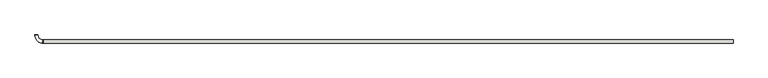
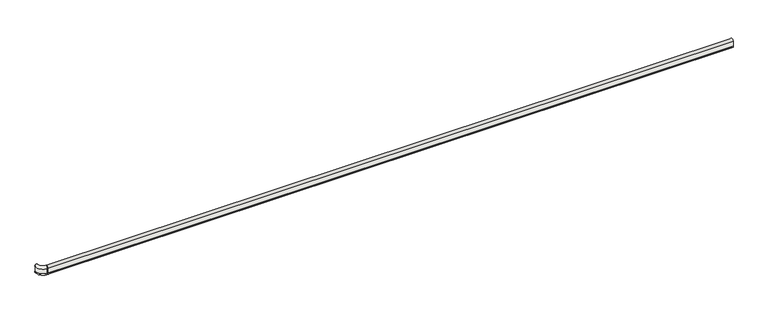
"""IFC4 building model written with IfcOpenShell, lengths in millimetres: covering geometry, Construction_Railing_SPM_Starline-Anodisee-Decowood : Decowood."""

import ifcopenshell
import ifcopenshell.guid

model = None  # the IFC model being written
_history = None  # IfcOwnerHistory: only IFC2X3 demands one
_inside = {}  # id of a spatial element -> (the spatial element, [elements in it])
_under = {}  # id of a project, library or spatial element -> (it, [spatial elements below it])
_declared = {}  # id of a project -> (the project, [libraries it declares])
_typed = {}  # id of a type object -> (the type object, [elements of that type])
_made_of = {}  # id of a material, layer set ... -> (it, [elements and type objects made of it])


def new_model(schema):
    """Start an empty IFC model of exactly this schema.

    Asked for "IFC4X3", IfcOpenShell would pick the latest addendum, in which some entities
    have other attributes; the version numbers below select the first issue.
    IFC2X3 requires an IfcOwnerHistory on every rooted entity: one is made here for all.
    """
    global model, _history
    if schema == "IFC4X3":
        model = ifcopenshell.file(schema_version=(4, 3, 0, 0))
    else:
        model = ifcopenshell.file(schema=schema)
    _inside.clear()
    _under.clear()
    _declared.clear()
    _typed.clear()
    _made_of.clear()
    _history = None
    if model.schema == "IFC2X3":
        org = make("IfcOrganization", Name="unknown")
        user = make(
            "IfcPersonAndOrganization",
            ThePerson=make("IfcPerson", FamilyName="unknown"),
            TheOrganization=org,
        )
        app = make(
            "IfcApplication",
            ApplicationDeveloper=org,
            Version="unknown",
            ApplicationFullName="unknown",
            ApplicationIdentifier="unknown",
        )
        _history = make(
            "IfcOwnerHistory",
            OwningUser=user,
            OwningApplication=app,
            ChangeAction="ADDED",
            CreationDate=0,
        )
    return model


def make(cls, **values):
    """One entity of the class cls with the attributes given. An attribute that is None is left unset."""
    return model.create_entity(
        cls, **{name: value for name, value in values.items() if value is not None}
    )


def rooted(cls, **values):
    """An entity with a GlobalId (a new one), such as an element, a storey or a relation."""
    return make(cls, GlobalId=ifcopenshell.guid.new(), OwnerHistory=_history, **values)


def si_unit(unit_type, name, prefix=None):
    """IfcSIUnit, for example si_unit("LENGTHUNIT", "METRE", prefix="MILLI")."""
    return make("IfcSIUnit", UnitType=unit_type, Prefix=prefix, Name=name)


def assignment(units):
    """IfcUnitAssignment: the units of a project."""
    return None if units is None else make("IfcUnitAssignment", Units=units)


def point(xyz):
    """IfcCartesianPoint."""
    return None if xyz is None else make("IfcCartesianPoint", Coordinates=xyz)


def direction(xyz):
    """IfcDirection."""
    return None if xyz is None else make("IfcDirection", DirectionRatios=xyz)


def frame(location, z_axis=None, x_axis=None):
    """IfcAxis2Placement3D, a coordinate frame: its origin and axes. An axis left out is left unset."""
    return make(
        "IfcAxis2Placement3D",
        Location=point(location),
        Axis=direction(z_axis),
        RefDirection=direction(x_axis),
    )


def frame_2d(location, x_axis=None):
    """IfcAxis2Placement2D, a coordinate frame in the plane: its origin and x axis."""
    return make(
        "IfcAxis2Placement2D", Location=point(location), RefDirection=direction(x_axis)
    )


def origin():
    """The frame at (0, 0, 0) with its axes left unset."""
    return frame((0.0, 0.0, 0.0))


def place(relative_to, where):
    """IfcLocalPlacement: puts the frame where relative to a parent placement (None: the world)."""
    return make(
        "IfcLocalPlacement", PlacementRelTo=relative_to, RelativePlacement=where
    )


def context(
    kind, dimensions, precision=None, world=None, true_north=None, identifier=None
):
    """IfcGeometricRepresentationContext, for example the 3D "Model" context."""
    return make(
        "IfcGeometricRepresentationContext",
        ContextIdentifier=identifier,
        ContextType=kind,
        CoordinateSpaceDimension=dimensions,
        Precision=precision,
        WorldCoordinateSystem=world,
        TrueNorth=true_north,
    )


def project(units=None, contexts=None):
    """IfcProject with its units and contexts."""
    return rooted(
        "IfcProject",
        Name="project",
        RepresentationContexts=contexts,
        UnitsInContext=assignment(units),
    )


def spatial(cls, under=None, at=None, **own):
    """A site, building, storey or space (cls), placed at a placement, below another one or the project."""
    s = rooted(cls, ObjectPlacement=at, **own)
    if under is not None:
        _under.setdefault(under.id(), (under, []))[1].append(s)
    return s


def polyline(points):
    """IfcPolyline through the points."""
    return make("IfcPolyline", Points=[point(p) for p in points])


def circle_curve(where, radius):
    """IfcCircle in the frame where."""
    return make("IfcCircle", Position=where, Radius=radius)


def ellipse_curve(where, semi_axis1, semi_axis2):
    """IfcEllipse in the frame where."""
    return make(
        "IfcEllipse", Position=where, SemiAxis1=semi_axis1, SemiAxis2=semi_axis2
    )


def trimmed(basis, trim1, trim2, sense, master):
    """IfcTrimmedCurve: the piece of a basis curve between two trims."""
    return make(
        "IfcTrimmedCurve",
        BasisCurve=basis,
        Trim1=trim1,
        Trim2=trim2,
        SenseAgreement=sense,
        MasterRepresentation=master,
    )


def segment(curve, same_sense, transition):
    """IfcCompositeCurveSegment."""
    return make(
        "IfcCompositeCurveSegment",
        Transition=transition,
        SameSense=same_sense,
        ParentCurve=curve,
    )


def composite_curve(segments, self_intersect=None):
    """IfcCompositeCurve: segments joined end to end."""
    return make("IfcCompositeCurve", Segments=segments, SelfIntersect=self_intersect)


def outline(outer, holes=None, kind="AREA"):
    """IfcArbitraryClosedProfileDef: a profile drawn as a closed curve; with holes, ...WithVoids."""
    if holes is None:
        return make("IfcArbitraryClosedProfileDef", ProfileType=kind, OuterCurve=outer)
    return make(
        "IfcArbitraryProfileDefWithVoids",
        ProfileType=kind,
        OuterCurve=outer,
        InnerCurves=holes,
    )


def extrude(swept, where, along, depth):
    """IfcExtrudedAreaSolid: the profile swept, set in the frame where, extruded along a direction by depth."""
    return make(
        "IfcExtrudedAreaSolid",
        SweptArea=swept,
        Position=where,
        ExtrudedDirection=direction(along),
        Depth=depth,
    )


def shape(context_of_items, identifier, shape_type, items):
    """IfcShapeRepresentation: the items that make up one representation, for example the "Body"."""
    return make(
        "IfcShapeRepresentation",
        ContextOfItems=context_of_items,
        RepresentationIdentifier=identifier,
        RepresentationType=shape_type,
        Items=items,
    )


def source(mapping_origin, context_of_items, identifier, shape_type, items):
    """IfcRepresentationMap: a shape defined once, which mapped items show again and again."""
    return make(
        "IfcRepresentationMap",
        MappingOrigin=mapping_origin,
        MappedRepresentation=shape(context_of_items, identifier, shape_type, items),
    )


def transform(
    local_origin,
    x_axis=None,
    y_axis=None,
    z_axis=None,
    scale=None,
    scale2=None,
    scale3=None,
    uniform=True,
):
    """IfcCartesianTransformationOperator3D, or its non-uniform kind. x_axis, y_axis, z_axis: its Axis1, 2, 3."""
    if uniform:
        return make(
            "IfcCartesianTransformationOperator3D",
            Axis1=direction(x_axis),
            Axis2=direction(y_axis),
            LocalOrigin=point(local_origin),
            Scale=scale,
            Axis3=direction(z_axis),
        )
    return make(
        "IfcCartesianTransformationOperator3DnonUniform",
        Axis1=direction(x_axis),
        Axis2=direction(y_axis),
        LocalOrigin=point(local_origin),
        Scale=scale,
        Axis3=direction(z_axis),
        Scale2=scale2,
        Scale3=scale3,
    )


def mapped(mapping_source, mapping_target):
    """IfcMappedItem: shows the shape of a source again, moved by a transform."""
    return make(
        "IfcMappedItem", MappingSource=mapping_source, MappingTarget=mapping_target
    )


def made_of(thing, what):
    """Note that an element or type object is made of a material, layer set ...; save() writes the relation."""
    if what is not None:
        _made_of.setdefault(what.id(), (what, []))[1].append(thing)
    return thing


def element(
    cls,
    number,
    at=None,
    inside=None,
    cuts=None,
    type_object=None,
    material=None,
    context=None,
    identifier="Body",
    shape_type=None,
    held_by="IfcProductDefinitionShape",
    body=None,
    shapes=None,
    **own,
):
    """One element of the class cls, such as IfcWall. Its Tag is "e" and its number.

    at: its placement. inside: the storey or other place that contains it. cuts: it is an
    opening in that element (IfcRelVoidsElement). A single representation is given by context,
    identifier, shape_type and body (its items); several are given by shapes. held_by: the class
    of the entity that holds the representations. save() writes the other relations.
    """
    e = rooted(cls, Tag="e%d" % number, ObjectPlacement=at, **own)
    if body is not None:
        shapes = [shape(context, identifier, shape_type, body)]
    if shapes is not None:
        e.Representation = make(held_by, Representations=shapes)
    if inside is not None:
        _inside.setdefault(inside.id(), (inside, []))[1].append(e)
    if cuts is not None:
        rooted(
            "IfcRelVoidsElement", RelatingBuildingElement=cuts, RelatedOpeningElement=e
        )
    if type_object is not None:
        _typed.setdefault(type_object.id(), (type_object, []))[1].append(e)
    return made_of(e, material)


def aggregate(whole, parts):
    """IfcRelAggregates: a whole, such as a stair, and the parts it consists of."""
    return rooted("IfcRelAggregates", RelatingObject=whole, RelatedObjects=parts)


def save(model, path):
    """Write the relations noted so far, then the file.

    IfcRelAggregates (storeys below a building ...), IfcRelContainedInSpatialStructure (elements
    in a storey), IfcRelDefinesByType, IfcRelAssociatesMaterial and IfcRelDeclares: one each for
    every whole, place, type object, material and project.
    """
    for whole, parts in _under.values():
        aggregate(whole, parts)
    for where, things in _inside.values():
        rooted(
            "IfcRelContainedInSpatialStructure",
            RelatedElements=things,
            RelatingStructure=where,
        )
    for kind, things in _typed.values():
        rooted("IfcRelDefinesByType", RelatedObjects=things, RelatingType=kind)
    for what, things in _made_of.values():
        rooted("IfcRelAssociatesMaterial", RelatedObjects=things, RelatingMaterial=what)
    for by, libraries in _declared.values():
        rooted("IfcRelDeclares", RelatingContext=by, RelatedDefinitions=libraries)
    model.write(path)


def plane_surface(at):
    """IfcPlane: the flat surface through the origin of the frame at, square to its z axis."""
    return make("IfcPlane", Position=at)


def cylinder_surface(at, radius):
    """IfcCylindricalSurface: all points at the distance radius from the z axis of the frame at."""
    return make("IfcCylindricalSurface", Position=at, Radius=radius)


def revolved_surface(curve, axis_point, axis_direction):
    """IfcSurfaceOfRevolution: the curve turned about the line through axis_point along axis_direction."""
    return make(
        "IfcSurfaceOfRevolution",
        SweptCurve=make("IfcArbitraryOpenProfileDef", ProfileType="CURVE", Curve=curve),
        AxisPosition=make("IfcAxis1Placement", Location=point(axis_point), Axis=direction(axis_direction)),
    )


def advanced_brep(points, edges, surfaces, faces):
    """IfcAdvancedBrep: a solid bounded by faces that lie on surfaces and meet in shared edges.

    An edge is (start, end): straight between two places in points (the first is 0);
    or (start, end, curve); or (start, end, curve, False) where it runs against its curve.
    A face is (place in surfaces, loops), or (place, loops, False) where it looks against
    its surface's normal. A loop lists edges by number (the first is 1), with a minus sign
    where the edge is run from its end to its start. The first loop is the outer one.
    """
    corners = [point(p) for p in points]
    vertices = [make("IfcVertexPoint", VertexGeometry=c) for c in corners]
    made = []
    for start, end, *more in edges:
        made.append(
            make(
                "IfcEdgeCurve",
                EdgeStart=vertices[start],
                EdgeEnd=vertices[end],
                EdgeGeometry=more[0] if more else make("IfcPolyline", Points=[corners[start], corners[end]]),
                SameSense=more[1] if len(more) > 1 else True,
            )
        )
    hull = []
    for where, loops, *sense in faces:
        bounds = []
        for j, loop in enumerate(loops):
            ring = [make("IfcOrientedEdge", EdgeElement=made[abs(k) - 1], Orientation=k > 0) for k in loop]
            bounds.append(
                make(
                    "IfcFaceOuterBound" if j == 0 else "IfcFaceBound",
                    Bound=make("IfcEdgeLoop", EdgeList=ring),
                    Orientation=True,
                )
            )
        hull.append(make("IfcAdvancedFace", Bounds=bounds, FaceSurface=surfaces[where], SameSense=sense[0] if sense else True))
    return make("IfcAdvancedBrep", Outer=make("IfcClosedShell", CfsFaces=hull))


def covering_4a841b85(model_context):
    return source(origin(), model_context, "Body", "SolidModel", [
        advanced_brep(
        [(0.0, -52.1949146, 777.1298269), (0.0, -78.97282, 779.8387167), (0.0, -77.7797808, 779.8387167), (0.0, -77.7797808, 730.187687), (0.0, -79.0444967, 730.187687), (0.0, -52.1949146, 732.7970729), (-1.0, -52.1949146, 777.1298269), (-1.0, -78.97282, 779.8387167), (-78.97282, -1.0, 779.8387167), (-78.97282, 0.0, 779.8387167), (-77.7797808, 0.0, 779.8387167), (-77.7797808, -1.0, 779.8387167), (-1.0, -77.7797808, 779.8387167), (-1.0, -77.7797808, 730.187687), (-77.7797808, -1.0, 730.187687), (-77.7797808, 0.0, 730.187687), (-79.0444967, 0.0, 730.187687), (-79.0444967, -1.0, 730.187687), (-1.0, -79.0444967, 730.187687), (-1.0, -52.1949146, 732.7970729), (-52.1949146, -1.0, 777.1298269), (-52.1949146, -1.0, 732.7970729), (-52.1949146, 0.0, 777.1298269), (-52.1949146, 0.0, 732.7970729)],
        [
            (0, 1, circle_curve(frame((0.0, -64.921376, 785.0331273), z_axis=(1.0, 0.0, 0.0), x_axis=(0.0, -1.0, 0.0)), 14.9808204)),
            (1, 2),
            (2, 3),
            (3, 4),
            (4, 5, circle_curve(frame((0.0, -64.9833199, 724.9442146), z_axis=(1.0, 0.0, 0.0), x_axis=(0.0, -1.0, 0.0)), 15.0070215)),
            (5, 0),
            (0, 6),
            (6, 7, circle_curve(frame((-1.0, -64.921376, 785.0331273), z_axis=(1.0, 0.0, 0.0), x_axis=(0.0, -1.0, 0.0)), 14.9808204)),
            (7, 1),
            (7, 8, circle_curve(frame((-1.0, -1.0, 779.8387167), z_axis=(0.0, 0.0, -1.0), x_axis=(0.0, -1.0, 0.0)), 77.97282)),
            (8, 9),
            (9, 10),
            (10, 11),
            (11, 12, circle_curve(frame((-1.0, -1.0, 779.8387167), z_axis=(0.0, 0.0, 1.0), x_axis=(0.0, -1.0, 0.0)), 76.7797808)),
            (12, 2),
            (12, 13),
            (13, 3),
            (13, 14, circle_curve(frame((-1.0, -1.0, 730.187687), z_axis=(0.0, 0.0, -1.0), x_axis=(0.0, -1.0, 0.0)), 76.7797808)),
            (14, 15),
            (15, 16),
            (16, 17),
            (17, 18, circle_curve(frame((-1.0, -1.0, 730.187687), z_axis=(0.0, 0.0, 1.0), x_axis=(0.0, -1.0, 0.0)), 78.0444967)),
            (18, 4),
            (18, 19, circle_curve(frame((-1.0, -64.9833199, 724.9442146), z_axis=(1.0, 0.0, 0.0), x_axis=(0.0, -1.0, 0.0)), 15.0070215)),
            (19, 5),
            (19, 6),
            (6, 20, circle_curve(frame((-1.0, -1.0, 777.1298269), z_axis=(0.0, 0.0, -1.0), x_axis=(0.0, -1.0, 0.0)), 51.1949146)),
            (20, 8, circle_curve(frame((-64.921376, -1.0, 785.0331273), z_axis=(0.0, -1.0, 0.0), x_axis=(-1.0, 0.0, 0.0)), 14.9808204)),
            (11, 14),
            (21, 19, circle_curve(frame((-1.0, -1.0, 732.7970729), z_axis=(0.0, 0.0, 1.0), x_axis=(0.0, -1.0, 0.0)), 51.1949146)),
            (17, 21, circle_curve(frame((-64.9833199, -1.0, 724.9442146), z_axis=(0.0, -1.0, 0.0), x_axis=(-1.0, 0.0, 0.0)), 15.0070215)),
            (21, 20),
            (22, 23),
            (23, 16, circle_curve(frame((-64.9833199, 0.0, 724.9442146), z_axis=(0.0, 1.0, 0.0), x_axis=(-1.0, 0.0, 0.0)), 15.0070215)),
            (15, 10),
            (9, 22, circle_curve(frame((-64.921376, 0.0, 785.0331273), z_axis=(0.0, 1.0, 0.0), x_axis=(-1.0, 0.0, 0.0)), 14.9808204)),
            (20, 22),
            (23, 21),
        ],
        [
            plane_surface(frame((0.0, -50.0, 710.0), z_axis=(1.0, 0.0, 0.0), x_axis=(0.0, 0.0, 1.0))),
            cylinder_surface(frame((0.0, -64.921376, 785.0331273), z_axis=(1.0, 0.0, 0.0), x_axis=(0.0, -1.0, 0.0)), 14.9808204),
            plane_surface(frame((0.0, -78.97282, 779.8387167), z_axis=(0.0, 0.0, -1.0), x_axis=(-1.0, 0.0, 0.0))),
            plane_surface(frame((0.0, -77.7797808, 779.8387167), z_axis=(0.0, -1.0, 0.0), x_axis=(-1.0, 0.0, 0.0))),
            plane_surface(frame((0.0, -77.7797808, 730.187687), z_axis=(0.0, 0.0, 1.0), x_axis=(-1.0, 0.0, 0.0))),
            cylinder_surface(frame((0.0, -64.9833199, 724.9442146), z_axis=(1.0, 0.0, 0.0), x_axis=(0.0, -1.0, 0.0)), 15.0070215),
            plane_surface(frame((0.0, -52.1949146, 732.7970729), z_axis=(0.0, 1.0, 0.0), x_axis=(-1.0, 0.0, 0.0))),
            revolved_surface(trimmed(ellipse_curve(frame((-1.0, -64.921376, 785.0331273), z_axis=(1.0, 0.0, 0.0), x_axis=(0.0, -1.0, 0.0)), 14.9808204, 14.9808204), [point((-1.0, -52.1949146, 777.1298269))], [point((-1.0, -78.97282, 779.8387167))], True, "CARTESIAN"), (-1.0, -1.0, 710.0), (0.0, 0.0, -1.0)),
            cylinder_surface(frame((-1.0, -1.0, 710.0), z_axis=(0.0, 0.0, -1.0), x_axis=(0.0, -1.0, 0.0)), 76.7797808),
            revolved_surface(trimmed(ellipse_curve(frame((-1.0, -64.9833199, 724.9442146), z_axis=(1.0, 0.0, 0.0), x_axis=(0.0, -1.0, 0.0)), 15.0070215, 15.0070215), [point((-1.0, -79.0444967, 730.187687))], [point((-1.0, -52.1949146, 732.7970729))], True, "CARTESIAN"), (-1.0, -1.0, 710.0), (0.0, 0.0, -1.0)),
            revolved_surface(polyline([(-1.0, -52.1949146, 732.7970729), (-1.0, -52.1949146, 777.1298269)]), (-1.0, -1.0, 710.0), (0.0, 0.0, -1.0)),
            plane_surface(frame((-50.0, 0.0, 710.0), z_axis=(0.0, 1.0, 0.0), x_axis=(0.0, 0.0, 1.0))),
            cylinder_surface(frame((-64.921376, -1.0, 785.0331273), z_axis=(0.0, -1.0, 0.0), x_axis=(-1.0, 0.0, 0.0)), 14.9808204),
            plane_surface(frame((-77.7797808, -1.0, 779.8387167), z_axis=(-1.0, 0.0, 0.0), x_axis=(0.0, 1.0, 0.0))),
            cylinder_surface(frame((-64.9833199, -1.0, 724.9442146), z_axis=(0.0, -1.0, 0.0), x_axis=(-1.0, 0.0, 0.0)), 15.0070215),
            plane_surface(frame((-52.1949146, -1.0, 732.7970729), z_axis=(1.0, 0.0, 0.0), x_axis=(0.0, 1.0, 0.0))),
        ],
        [
            (0, [[1, 2, 3, 4, 5, 6]]),
            (1, [[-1, 7, 8, 9]]),
            (2, [[-2, -9, 10, 11, 12, 13, 14, 15]]),
            (3, [[-3, -15, 16, 17]]),
            (4, [[-4, -17, 18, 19, 20, 21, 22, 23]]),
            (5, [[-5, -23, 24, 25]]),
            (6, [[-6, -25, 26, -7]]),
            (7, [[-10, -8, 27, 28]]),
            (8, [[-18, -16, -14, 29]]),
            (9, [[30, -24, -22, 31]]),
            (10, [[-27, -26, -30, 32]]),
            (11, [[33, 34, -20, 35, -12, 36]]),
            (12, [[-28, 37, -36, -11]]),
            (13, [[-29, -13, -35, -19]]),
            (14, [[-31, -21, -34, 38]]),
            (15, [[-32, -38, -33, -37]]),
        ],
    ),
        extrude(outline(composite_curve([segment(trimmed(circle_curve(frame_2d((-64.921376, 785.0331273)), 14.9808204), [point((-78.97282, 779.8387167))], [point((-52.1949146, 777.1298269))], False, "CARTESIAN"), True, "CONTINUOUS"), segment(polyline([(-52.1949146, 777.1298269), (-52.1949146, 732.7970729)]), True, "CONTINUOUS"), segment(trimmed(circle_curve(frame_2d((-64.9833199, 724.9442146)), 15.0070215), [point((-52.1949146, 732.7970729))], [point((-79.0444967, 730.187687))], False, "CARTESIAN"), True, "CONTINUOUS"), segment(polyline([(-79.0444967, 730.187687), (-77.7797808, 730.187687), (-77.7797808, 779.8387167), (-78.97282, 779.8387167)]), True, "CONTINUOUS")], self_intersect=False)), frame((0.0, 0.0, 0.0), z_axis=(1.0, 0.0, 0.0), x_axis=(0.0, 1.0, 0.0)), (0.0, 0.0, 1.0), 6800.0),
        extrude(outline(polyline([(0.0, -79.3173438), (0.0, -77.7797808), (6800.0, -77.7797808), (6800.0, -79.3173438), (0.0, -79.3173438)])), frame((0.0, 0.0, 730.187687), z_axis=(0.0, 0.0, 1.0), x_axis=(1.0, 0.0, 0.0)), (0.0, 0.0, 1.0), 49.6510297),
    ])


if __name__ == "__main__":
    model = new_model("IFC4")
    model_context = context("Model", 3, world=origin())
    ifc_project = project(units=[si_unit("LENGTHUNIT", "METRE", prefix="MILLI")], contexts=[model_context])
    site = spatial("IfcSite", under=ifc_project)
    building = spatial("IfcBuilding", under=site)
    placement = place(None, origin())
    covering_shape = covering_4a841b85(model_context)
    element("IfcCovering", 1, ObjectType="Construction_Railing_SPM_Starline-Anodisee-Decowood : Decowood", at=placement, inside=building, context=model_context, shape_type="MappedRepresentation", body=[
        mapped(covering_shape, transform((0.0, 0.0, 0.0), x_axis=(1.0, 0.0, 0.0), y_axis=(0.0, 1.0, 0.0), z_axis=(0.0, 0.0, 1.0))),
    ])
    save(model, "model.ifc")

# Revit data of these elements
# Type "Construction_Railing_SPM_Starline-Anodisee-Decowood : Decowood"
#   WarrantyStartDate [instance default] = "1900-12-31T23:59:59"
#   WarrantyGuarantorParts = "n/a"
#   WarrantyGuarantorLabor = "n/a"
#   WarrantyDurationUnit = "year"
#   WarrantyDurationParts = "n/a"
#   WarrantyDurationLabor = "n/a"
#   WarrantyDescription = "n/a"
#   WallStandoff = "50 mm"
#   URL = "www.spm.fr"
#   UNSPSC Code = ""
#   TagNumber [instance default] = "n/a"
#   SustainabilityPerformance = "n/a"
#   SurfaceSpreadOfFlame = "n/a"
#   Size = "90 x 80 x 4000 mm"
#   Shape = "Elliptical"
#   SerialNumber [instance default] = "n/a"
#   ReplacementCost = "n/a"
#   Reference = "n/a"
#   Projection = "80 mm"
#   Product data url = "http://bimobject.com/spm/product/SPM-STARLINE-DECO"
#   Product Guid = "a7a4224a-4578-432f-a478-06146786615d"
#   OmniClass Description = ""
#   OmniClass Code = ""
#   Name = "WallProtectionPanels_StarlineDecowoodHandrail_GerflorLtd"
#   NBS Reference Description = ""
#   NBS Reference Code = ""
#   ModelReference = "Starline Decowood Handrail"
#   ModelNumber = "n/a"
#   Model = "Starline Decowood Handrail"
#   Material secondary = ""
#   Material main = ""
#   Material = "1.5 mm thick aluminium"
#   Manufacturer = "SPM"
#   Keynote = "09100"
#   InstallationDate [instance default] = "1900-12-31T23:59:59"
#   IfcExportType = "NOTDEFINED"
#   IfcExportAs = "IfcCoveringType"
#   IFC Classification = ""
#   Grade = "n/a"
#   FragilityRating = "n/a"
#   FlammabilityRating = "n/a"
#   Fixing = "2-point self-locking perforated satin silver anodized aluminium brackets"
#   FireRating = "B-s2, d0"
#   Finish = "Aluminium profile: Satin silver anodized; PVC band: Wood effect"
#   Features = "Excellent wrenching resistance, antibacterial"
#   ExpectedLife = "n/a"
#   EnvironmentalProductDeclaration = "n/a"
#   EAN code = ""
#   DurationUnit = "year"
#   Description = "Range only available for the French market"
#   CrossSection = "Elliptical"
#   Constituents = "n/a"
#   ColourOptions = "PVC band: 7 wood effect and 2 trend effect colours available"
#   Color = "n/a"
#   CodePerformance = "n/a"
#   Category = "n/a"
#   COBIe Type Category = ""
#   BarCode [instance default] = "n/a"
#   BIMobject category = ""
#   AssetType = "Fixed"
#   AssetIdentifier [instance default] = "n/a"
#   Assembly Code = "C10"
#   Applications = "Straight and curved corridors in public buildings such as hospitals, clinics, retirement homes, hotels and offices"
#   AcousticRating = "n/a"
#   Accessories = "90° external angle pieces, Variable angles, Wall returns"
#   AccessibilityPerformance = "n/a"
#   Width = 80 mm
#   TotalThickness = 80 mm
#   SpacerOffsetRight [instance default] = 100 mm
#   SpacerOffsetLeft [instance default] = 100 mm
#   OffsetFromWall = 50 mm
#   NominalLength [instance default] = 4000 mm
#   Height = 90 mm
#   HandrailHeight [instance default] = 800 mm
#   SpacerVerticalPlacement [instance default] = 724 mm
#   SpacerCentreToCentreDistance [instance default] = 950 mm
#   SpacerCalc [instance default] = 3800 mm
#   SpacerOffsetRightControl [instance default] = 100 mm
#   SpacerOffsetLeftControl [instance default] = 100 mm
#   MaximumSpacerCentreDistance [instance default] = 1200 mm
#   built-in parameter 1001306 [instance default] = 13.1234 (stored number, unit not read)
#   Diameter = 0 mm
#   Depth = 80 mm
#   NumberOfStandardRailLengths [instance default] = 1
#   NumberOfSpacers [instance default] = 5
#   IsExternal = no
#   HasHeavyTraffic [instance default] = no
#   Edition number = 1
#   CrashRailInternalCornerRight [instance default] = no
#   CrashRailInternalCornerLeft [instance default] = no
#   CrashRailExternalCornerRight [instance default] = yes
#   CrashRailExternalCornerLeft [instance default] = yes
#   CrashRailEndCapRight [instance default] = no
#   CrashRailEndCapLeft [instance default] = no
#   Combustible = no
#   InsertMaterial = PVC - SPM - Erable
#   SpacerMaterial = PVC - SPM - Hêtre
#   RailMaterial = PVC - SPM - Wengé
#   Default Elevation = 0
#   Cost = 0
# Element 1 (IfcCovering, "Construction_Railing_SPM_Starline-Anodisee-Decowood : Decowood")
#   NominalLength = 6800 mm
#   SpacerCentreToCentreDistance = 1100 mm
#   SpacerCalc = 6600 mm
#   built-in parameter 1001306 = 22.3097 (stored number, unit not read)
#   NumberOfStandardRailLengths = 2
#   NumberOfSpacers = 7
#   Materials on its faces: "PVC - SPM - Wengé", "PVC - SPM - Erable"
# Materials
#   "PVC - SPM - Erable": class "Plastique", colour RGB 155 148 134, transparency 0, Keynote = "09700", Model = "0060 Erable", Manufacturer = "SPM", URL = "www.spm.fr", Description = "Gamme Bois", Cost = 0
#   "PVC - SPM - Hêtre": class "Plastique", colour RGB 140 126 100, transparency 0, Keynote = "09700", Model = "0061 Hêtre", Manufacturer = "SPM", URL = "www.spm.fr", Description = "Gamme Bois", Cost = 0
#   "PVC - SPM - Wengé": class "Plastique", colour RGB 64 50 47, transparency 0, Keynote = "09700", Model = "0067 Wengé", Manufacturer = "SPM", URL = "www.spm.fr", Description = "Gamme Bois", Cost = 0
